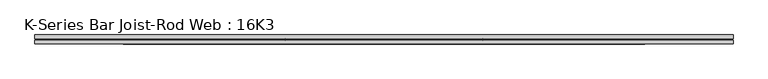
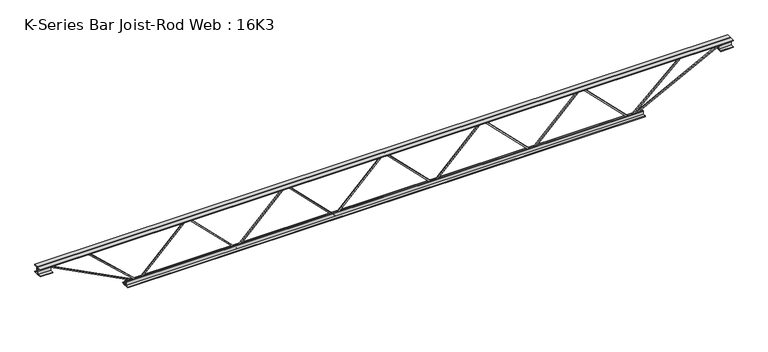
"""IFC4 building model written with IfcOpenShell, lengths in millimetres: beam geometry, K-Series Bar Joist-Rod Web : 16K3."""

from ifc_helpers import new_model, si_unit, frame, origin, place, context, project, spatial, polyline, outline, extrude, source, transform, mapped, element, save


def k_series_bar_joist_rod_web_16k3_8f8c8369(model_context):
    return source(origin(), model_context, "Body", "SweptSolid", [
        extrude(outline(polyline([(-192.0875, 398.78), (-201.6125, 398.78), (-201.6125, 403.9322006), (192.0875, 796.3622006), (192.0875, 798.7577994), (-201.6125, 1191.1877994), (-201.6125, 1196.34), (-192.0875, 1196.34), (-192.0875, 1195.1422006), (201.6125, 802.7122006), (201.6125, 792.4077994), (-192.0875, 399.9777994), (-192.0875, 398.78)])), frame((0.0, -4.7625, 0.0), z_axis=(0.0, 1.0, 0.0), x_axis=(0.0, 0.0, 1.0)), (0.0, 0.0, 1.0), 9.525),
        extrude(outline(polyline([(-192.0875, -398.78), (-201.6125, -398.78), (-201.6125, -393.6277994), (192.0875, -1.1977994), (192.0875, 1.1977994), (-201.6125, 393.6277994), (-201.6125, 398.78), (-192.0875, 398.78), (-192.0875, 397.5822006), (201.6125, 5.1522006), (201.6125, -5.1522006), (-192.0875, -397.5822006), (-192.0875, -398.78)])), frame((0.0, -4.7625, 0.0), z_axis=(0.0, 1.0, 0.0), x_axis=(0.0, 0.0, 1.0)), (0.0, 0.0, 1.0), 9.525),
        extrude(outline(polyline([(-192.0875, -1196.34), (-201.6125, -1196.34), (-201.6125, -1191.1877994), (192.0875, -798.7577994), (192.0875, -796.3622006), (-201.6125, -403.9322006), (-201.6125, -398.78), (-192.0875, -398.78), (-192.0875, -399.9777994), (201.6125, -792.4077994), (201.6125, -802.7122006), (-192.0875, -1195.1422006), (-192.0875, -1196.34)])), frame((0.0, -4.7625, 0.0), z_axis=(0.0, 1.0, 0.0), x_axis=(0.0, 0.0, 1.0)), (0.0, 0.0, 1.0), 9.525),
        extrude(outline(polyline([(-192.0875, 1196.34), (-201.6125, 1196.34), (-201.6125, 1201.4922006), (192.0875, 1593.9222006), (192.0875, 1596.3177994), (-201.6125, 1988.7477994), (-201.6125, 1993.9), (-192.0875, 1993.9), (-192.0875, 1992.7022006), (201.6125, 1600.2722006), (201.6125, 1589.9677994), (-192.0875, 1197.5377994), (-192.0875, 1196.34)])), frame((0.0, -4.7625, 0.0), z_axis=(0.0, 1.0, 0.0), x_axis=(0.0, 0.0, 1.0)), (0.0, 0.0, 1.0), 9.525),
        extrude(outline(polyline([(-192.0875, -1993.9), (-201.6125, -1993.9), (-201.6125, -1988.7477994), (192.0875, -1596.3177994), (192.0875, -1593.9222006), (-201.6125, -1201.4922006), (-201.6125, -1196.34), (-192.0875, -1196.34), (-192.0875, -1197.5377994), (201.6125, -1589.9677994), (201.6125, -1600.2722006), (-192.0875, -1992.7022006), (-192.0875, -1993.9)])), frame((0.0, -4.7625, 0.0), z_axis=(0.0, 1.0, 0.0), x_axis=(0.0, 0.0, 1.0)), (0.0, 0.0, 1.0), 9.525),
        extrude(outline(polyline([(4.7625, 203.2), (36.5125, 203.2), (36.5125, 196.85), (11.1125, 196.85), (11.1125, 171.45), (4.7625, 171.45), (4.7625, 203.2)])), frame((-2806.7, 0.0, 0.0), z_axis=(1.0, 0.0, 0.0), x_axis=(0.0, 1.0, 0.0)), (0.0, 0.0, 1.0), 5613.4),
        extrude(outline(polyline([(-4.7625, 203.2), (-4.7625, 171.45), (-11.1125, 171.45), (-11.1125, 196.85), (-36.5125, 196.85), (-36.5125, 203.2), (-4.7625, 203.2)])), frame((-2806.7, 0.0, 0.0), z_axis=(1.0, 0.0, 0.0), x_axis=(0.0, 1.0, 0.0)), (0.0, 0.0, 1.0), 5613.4),
        extrude(outline(polyline([(-4.7625, 139.7), (-36.5125, 139.7), (-36.5125, 146.05), (-11.1125, 146.05), (-11.1125, 171.45), (-4.7625, 171.45), (-4.7625, 139.7)])), frame((-2806.7, 0.0, 0.0), z_axis=(1.0, 0.0, 0.0), x_axis=(0.0, 1.0, 0.0)), (0.0, 0.0, 1.0), 101.6),
        extrude(outline(polyline([(36.5125, 139.7), (4.7625, 139.7), (4.7625, 171.45), (11.1125, 171.45), (11.1125, 146.05), (36.5125, 146.05), (36.5125, 139.7)])), frame((-2806.7, 0.0, 0.0), z_axis=(1.0, 0.0, 0.0), x_axis=(0.0, 1.0, 0.0)), (0.0, 0.0, 1.0), 101.6),
        extrude(outline(polyline([(4.7625, 139.7), (4.7625, 171.45), (11.1125, 171.45), (11.1125, 146.05), (36.5125, 146.05), (36.5125, 139.7), (4.7625, 139.7)])), frame((2705.1, 0.0, 0.0), z_axis=(1.0, 0.0, 0.0), x_axis=(0.0, 1.0, 0.0)), (0.0, 0.0, 1.0), 101.6),
        extrude(outline(polyline([(-4.7625, 139.7), (-36.5125, 139.7), (-36.5125, 146.05), (-11.1125, 146.05), (-11.1125, 171.45), (-4.7625, 171.45), (-4.7625, 139.7)])), frame((2705.1, 0.0, 0.0), z_axis=(1.0, 0.0, 0.0), x_axis=(0.0, 1.0, 0.0)), (0.0, 0.0, 1.0), 101.6),
        extrude(outline(polyline([(4.7625, -203.2), (4.7625, -171.45), (11.1125, -171.45), (11.1125, -196.85), (36.5125, -196.85), (36.5125, -203.2), (4.7625, -203.2)])), frame((-2095.5, 0.0, 0.0), z_axis=(1.0, 0.0, 0.0), x_axis=(0.0, 1.0, 0.0)), (0.0, 0.0, 1.0), 4191.0),
        extrude(outline(polyline([(-4.7625, -203.2), (-36.5125, -203.2), (-36.5125, -196.85), (-11.1125, -196.85), (-11.1125, -171.45), (-4.7625, -171.45), (-4.7625, -203.2)])), frame((-2095.5, 0.0, 0.0), z_axis=(1.0, 0.0, 0.0), x_axis=(0.0, 1.0, 0.0)), (0.0, 0.0, 1.0), 4191.0),
        extrude(outline(polyline([(0.0, -9.525), (0.0, 0.0), (800.9059433, 0.0), (800.9059433, -9.525), (0.0, -9.525)])), frame((-2707.2900559, 4.7625, 167.2209266), z_axis=(0.45985424766113664, 0.0, 0.8879944092774514), x_axis=(0.8879944092774514, 0.0, -0.45985424766113664)), (0.0, 0.0, 1.0), 9.525),
        extrude(outline(polyline([(0.0, -9.525), (0.0, 0.0), (542.8354985, 0.0), (542.8354985, -9.525), (0.0, -9.525)])), frame((-2395.9112344, 4.7625, 167.9513531), z_axis=(0.6784744200358839, 0.0, 0.7346240272118596), x_axis=(0.7346240272118596, 0.0, -0.6784744200358839)), (0.0, 0.0, 1.0), 9.525),
        extrude(outline(polyline([(0.0, -9.525), (0.0, 0.0), (800.9059433, 0.0), (800.9059433, -9.525), (0.0, -9.525)])), frame((2707.2900559, -4.7625, 167.2209266), z_axis=(-0.4598542476611243, 0.0, 0.8879944092774579), x_axis=(-0.8879944092774579, 0.0, -0.4598542476611243)), (0.0, 0.0, 1.0), 9.525),
        extrude(outline(polyline([(0.0, -9.525), (0.0, 0.0), (542.8354985, 0.0), (542.8354985, -9.525), (0.0, -9.525)])), frame((2395.9112344, -4.7625, 167.9513531), z_axis=(-0.6784744200358788, 0.0, 0.7346240272118643), x_axis=(-0.7346240272118643, 0.0, -0.6784744200358788)), (0.0, 0.0, 1.0), 9.525),
    ])


if __name__ == "__main__":
    model = new_model("IFC4")
    model_context = context("Model", 3, world=origin())
    ifc_project = project(units=[si_unit("LENGTHUNIT", "METRE", prefix="MILLI")], contexts=[model_context])
    site = spatial("IfcSite", under=ifc_project)
    building = spatial("IfcBuilding", under=site)
    placement = place(None, origin())
    k_series_bar_joist_rod_web_16k3_shape = k_series_bar_joist_rod_web_16k3_8f8c8369(model_context)
    element("IfcBeam", 1, ObjectType="K-Series Bar Joist-Rod Web : 16K3", at=placement, inside=building, context=model_context, shape_type="MappedRepresentation", body=[
        mapped(k_series_bar_joist_rod_web_16k3_shape, transform((0.0, 0.0, 0.0), x_axis=(1.0, 0.0, 0.0), y_axis=(0.0, 1.0, 0.0), z_axis=(0.0, 0.0, 1.0))),
    ])
    save(model, "model.ifc")

# Revit data of these elements
# Type "K-Series Bar Joist-Rod Web : 16K3"
#   Assembly Code = "B1010350"
#   Wt = 6.3
#   Web Thickness = 0' - 0 3/8"
#   Start Offset [instance default] = 0' - 0"
#   Start Extension [instance default] = 0' - 0"
#   Seat Length = 0' - 4"
#   Seat Depth = 0' - 2 1/2"
#   PanelArrayLength [instance default] = 18' - 8"
#   Panel [instance default] = 2' - 8"
#   End Offset [instance default] = 0' - 0"
#   End Extension [instance default] = 0' - 0"
#   End Panel = 2' - 8"
#   Cord Leg = 0' - 1 1/4"
#   Chord Thickness = 0' - 0 1/4"
#   Length [instance default] = 24' - 0"
#   Depth = 1' - 4"
#   PanelArrayNum [instance default] = 7
#   Structural Material = none
# Element 1 (IfcBeam, "K-Series Bar Joist-Rod Web : 16K3")
#   PanelArrayLength = 13' - 1"
#   Panel = 2' - 7.4"
#   PanelArrayNum = 5
